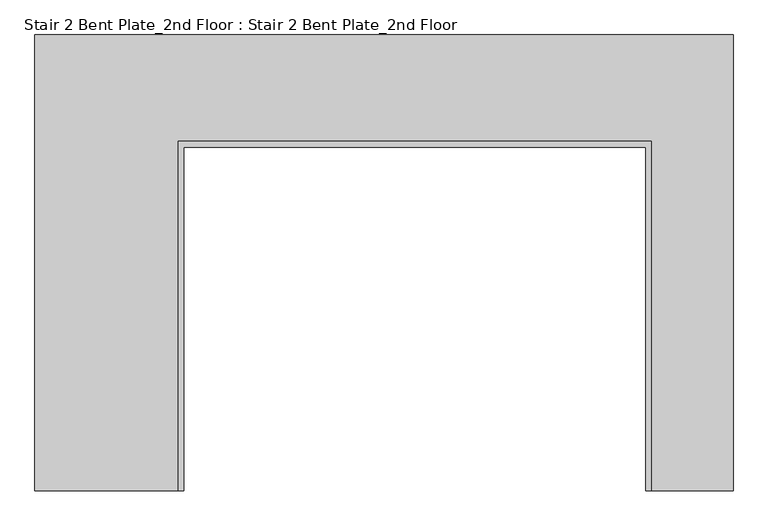
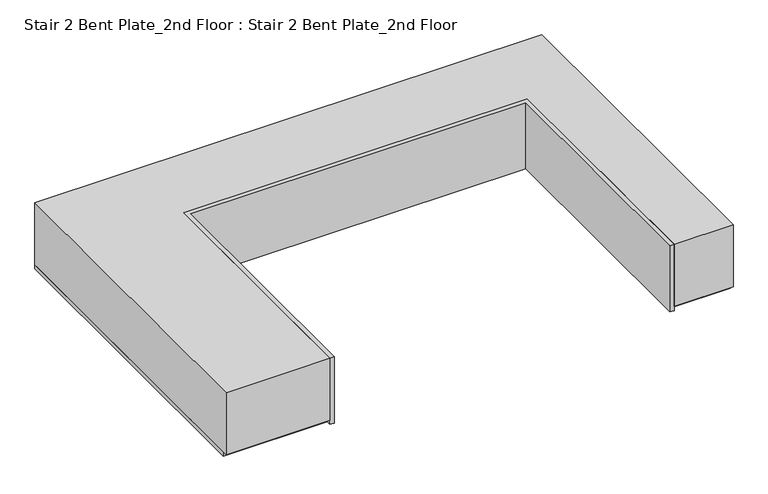
"""IFC4 building model written with IfcOpenShell, lengths in millimetres: proxy geometry, Stair 2 Bent Plate_2nd Floor : Stair 2 Bent Plate_2nd Floor."""

import ifcopenshell
import ifcopenshell.guid

model = None  # the IFC model being written
_history = None  # IfcOwnerHistory: only IFC2X3 demands one
_inside = {}  # id of a spatial element -> (the spatial element, [elements in it])
_under = {}  # id of a project, library or spatial element -> (it, [spatial elements below it])
_declared = {}  # id of a project -> (the project, [libraries it declares])
_typed = {}  # id of a type object -> (the type object, [elements of that type])
_made_of = {}  # id of a material, layer set ... -> (it, [elements and type objects made of it])


def new_model(schema):
    """Start an empty IFC model of exactly this schema.

    Asked for "IFC4X3", IfcOpenShell would pick the latest addendum, in which some entities
    have other attributes; the version numbers below select the first issue.
    IFC2X3 requires an IfcOwnerHistory on every rooted entity: one is made here for all.
    """
    global model, _history
    if schema == "IFC4X3":
        model = ifcopenshell.file(schema_version=(4, 3, 0, 0))
    else:
        model = ifcopenshell.file(schema=schema)
    _inside.clear()
    _under.clear()
    _declared.clear()
    _typed.clear()
    _made_of.clear()
    _history = None
    if model.schema == "IFC2X3":
        org = make("IfcOrganization", Name="unknown")
        user = make(
            "IfcPersonAndOrganization",
            ThePerson=make("IfcPerson", FamilyName="unknown"),
            TheOrganization=org,
        )
        app = make(
            "IfcApplication",
            ApplicationDeveloper=org,
            Version="unknown",
            ApplicationFullName="unknown",
            ApplicationIdentifier="unknown",
        )
        _history = make(
            "IfcOwnerHistory",
            OwningUser=user,
            OwningApplication=app,
            ChangeAction="ADDED",
            CreationDate=0,
        )
    return model


def make(cls, **values):
    """One entity of the class cls with the attributes given. An attribute that is None is left unset."""
    return model.create_entity(
        cls, **{name: value for name, value in values.items() if value is not None}
    )


def rooted(cls, **values):
    """An entity with a GlobalId (a new one), such as an element, a storey or a relation."""
    return make(cls, GlobalId=ifcopenshell.guid.new(), OwnerHistory=_history, **values)


def si_unit(unit_type, name, prefix=None):
    """IfcSIUnit, for example si_unit("LENGTHUNIT", "METRE", prefix="MILLI")."""
    return make("IfcSIUnit", UnitType=unit_type, Prefix=prefix, Name=name)


def assignment(units):
    """IfcUnitAssignment: the units of a project."""
    return None if units is None else make("IfcUnitAssignment", Units=units)


def point(xyz):
    """IfcCartesianPoint."""
    return None if xyz is None else make("IfcCartesianPoint", Coordinates=xyz)


def direction(xyz):
    """IfcDirection."""
    return None if xyz is None else make("IfcDirection", DirectionRatios=xyz)


def frame(location, z_axis=None, x_axis=None):
    """IfcAxis2Placement3D, a coordinate frame: its origin and axes. An axis left out is left unset."""
    return make(
        "IfcAxis2Placement3D",
        Location=point(location),
        Axis=direction(z_axis),
        RefDirection=direction(x_axis),
    )


def origin():
    """The frame at (0, 0, 0) with its axes left unset."""
    return frame((0.0, 0.0, 0.0))


def origin_with_axes():
    """The frame at (0, 0, 0) with the z axis (0, 0, 1) and the x axis (1, 0, 0) written out."""
    return frame((0.0, 0.0, 0.0), z_axis=(0.0, 0.0, 1.0), x_axis=(1.0, 0.0, 0.0))


def place(relative_to, where):
    """IfcLocalPlacement: puts the frame where relative to a parent placement (None: the world)."""
    return make(
        "IfcLocalPlacement", PlacementRelTo=relative_to, RelativePlacement=where
    )


def context(
    kind, dimensions, precision=None, world=None, true_north=None, identifier=None
):
    """IfcGeometricRepresentationContext, for example the 3D "Model" context."""
    return make(
        "IfcGeometricRepresentationContext",
        ContextIdentifier=identifier,
        ContextType=kind,
        CoordinateSpaceDimension=dimensions,
        Precision=precision,
        WorldCoordinateSystem=world,
        TrueNorth=true_north,
    )


def project(units=None, contexts=None):
    """IfcProject with its units and contexts."""
    return rooted(
        "IfcProject",
        Name="project",
        RepresentationContexts=contexts,
        UnitsInContext=assignment(units),
    )


def spatial(cls, under=None, at=None, **own):
    """A site, building, storey or space (cls), placed at a placement, below another one or the project."""
    s = rooted(cls, ObjectPlacement=at, **own)
    if under is not None:
        _under.setdefault(under.id(), (under, []))[1].append(s)
    return s


def polyline(points):
    """IfcPolyline through the points."""
    return make("IfcPolyline", Points=[point(p) for p in points])


def outline(outer, holes=None, kind="AREA"):
    """IfcArbitraryClosedProfileDef: a profile drawn as a closed curve; with holes, ...WithVoids."""
    if holes is None:
        return make("IfcArbitraryClosedProfileDef", ProfileType=kind, OuterCurve=outer)
    return make(
        "IfcArbitraryProfileDefWithVoids",
        ProfileType=kind,
        OuterCurve=outer,
        InnerCurves=holes,
    )


def extrude(swept, where, along, depth):
    """IfcExtrudedAreaSolid: the profile swept, set in the frame where, extruded along a direction by depth."""
    return make(
        "IfcExtrudedAreaSolid",
        SweptArea=swept,
        Position=where,
        ExtrudedDirection=direction(along),
        Depth=depth,
    )


def shape(context_of_items, identifier, shape_type, items):
    """IfcShapeRepresentation: the items that make up one representation, for example the "Body"."""
    return make(
        "IfcShapeRepresentation",
        ContextOfItems=context_of_items,
        RepresentationIdentifier=identifier,
        RepresentationType=shape_type,
        Items=items,
    )


def source(mapping_origin, context_of_items, identifier, shape_type, items):
    """IfcRepresentationMap: a shape defined once, which mapped items show again and again."""
    return make(
        "IfcRepresentationMap",
        MappingOrigin=mapping_origin,
        MappedRepresentation=shape(context_of_items, identifier, shape_type, items),
    )


def transform(
    local_origin,
    x_axis=None,
    y_axis=None,
    z_axis=None,
    scale=None,
    scale2=None,
    scale3=None,
    uniform=True,
):
    """IfcCartesianTransformationOperator3D, or its non-uniform kind. x_axis, y_axis, z_axis: its Axis1, 2, 3."""
    if uniform:
        return make(
            "IfcCartesianTransformationOperator3D",
            Axis1=direction(x_axis),
            Axis2=direction(y_axis),
            LocalOrigin=point(local_origin),
            Scale=scale,
            Axis3=direction(z_axis),
        )
    return make(
        "IfcCartesianTransformationOperator3DnonUniform",
        Axis1=direction(x_axis),
        Axis2=direction(y_axis),
        LocalOrigin=point(local_origin),
        Scale=scale,
        Axis3=direction(z_axis),
        Scale2=scale2,
        Scale3=scale3,
    )


def mapped(mapping_source, mapping_target):
    """IfcMappedItem: shows the shape of a source again, moved by a transform."""
    return make(
        "IfcMappedItem", MappingSource=mapping_source, MappingTarget=mapping_target
    )


def made_of(thing, what):
    """Note that an element or type object is made of a material, layer set ...; save() writes the relation."""
    if what is not None:
        _made_of.setdefault(what.id(), (what, []))[1].append(thing)
    return thing


def element(
    cls,
    number,
    at=None,
    inside=None,
    cuts=None,
    type_object=None,
    material=None,
    context=None,
    identifier="Body",
    shape_type=None,
    held_by="IfcProductDefinitionShape",
    body=None,
    shapes=None,
    **own,
):
    """One element of the class cls, such as IfcWall. Its Tag is "e" and its number.

    at: its placement. inside: the storey or other place that contains it. cuts: it is an
    opening in that element (IfcRelVoidsElement). A single representation is given by context,
    identifier, shape_type and body (its items); several are given by shapes. held_by: the class
    of the entity that holds the representations. save() writes the other relations.
    """
    e = rooted(cls, Tag="e%d" % number, ObjectPlacement=at, **own)
    if body is not None:
        shapes = [shape(context, identifier, shape_type, body)]
    if shapes is not None:
        e.Representation = make(held_by, Representations=shapes)
    if inside is not None:
        _inside.setdefault(inside.id(), (inside, []))[1].append(e)
    if cuts is not None:
        rooted(
            "IfcRelVoidsElement", RelatingBuildingElement=cuts, RelatedOpeningElement=e
        )
    if type_object is not None:
        _typed.setdefault(type_object.id(), (type_object, []))[1].append(e)
    return made_of(e, material)


def aggregate(whole, parts):
    """IfcRelAggregates: a whole, such as a stair, and the parts it consists of."""
    return rooted("IfcRelAggregates", RelatingObject=whole, RelatedObjects=parts)


def save(model, path):
    """Write the relations noted so far, then the file.

    IfcRelAggregates (storeys below a building ...), IfcRelContainedInSpatialStructure (elements
    in a storey), IfcRelDefinesByType, IfcRelAssociatesMaterial and IfcRelDeclares: one each for
    every whole, place, type object, material and project.
    """
    for whole, parts in _under.values():
        aggregate(whole, parts)
    for where, things in _inside.values():
        rooted(
            "IfcRelContainedInSpatialStructure",
            RelatedElements=things,
            RelatingStructure=where,
        )
    for kind, things in _typed.values():
        rooted("IfcRelDefinesByType", RelatedObjects=things, RelatingType=kind)
    for what, things in _made_of.values():
        rooted("IfcRelAssociatesMaterial", RelatedObjects=things, RelatingMaterial=what)
    for by, libraries in _declared.values():
        rooted("IfcRelDeclares", RelatingContext=by, RelatedDefinitions=libraries)
    model.write(path)


def stair_2_bent_plate_2nd_floor_stair_2_bent_plate_2nd_floor_d30ef73d(model_context):
    return source(origin(), model_context, "Body", "SweptSolid", [
        extrude(outline(polyline([(-314.325, -915.9875), (-314.325, 46.0375), (1158.875, 46.0375), (1158.875, -915.9875), (987.425, -915.9875), (987.425, -177.8), (-12.7, -177.8), (-12.7, -915.9875), (-314.325, -915.9875)])), frame((0.0, 0.0, 12.7), z_axis=(0.0, 0.0, 1.0), x_axis=(1.0, 0.0, 0.0)), (0.0, 0.0, 1.0), 190.5),
        extrude(outline(polyline([(-12.7, -901.7), (-314.325, -901.7), (-314.325, 46.0375), (1158.875, 46.0375), (1158.875, -901.7), (987.425, -901.7), (987.425, -177.8), (-12.7, -177.8), (-12.7, -901.7)])), origin_with_axes(), (0.0, 0.0, 1.0), 12.7),
        extrude(outline(polyline([(-12.7, -915.9875), (-12.7, -190.5), (-12.7, -177.8), (974.725, -177.8), (987.425, -177.8), (987.425, -915.9875), (974.725, -915.9875), (974.725, -190.5), (0.0, -190.5), (0.0, -915.9875), (-12.7, -915.9875)])), origin_with_axes(), (0.0, 0.0, 1.0), 203.2),
    ])


if __name__ == "__main__":
    model = new_model("IFC4")
    model_context = context("Model", 3, world=origin())
    ifc_project = project(units=[si_unit("LENGTHUNIT", "METRE", prefix="MILLI")], contexts=[model_context])
    site = spatial("IfcSite", under=ifc_project)
    building = spatial("IfcBuilding", under=site)
    placement = place(None, origin())
    stair_2_bent_plate_2nd_floor_stair_2_bent_plate_2nd_floor_shape = stair_2_bent_plate_2nd_floor_stair_2_bent_plate_2nd_floor_d30ef73d(model_context)
    element("IfcBuildingElementProxy", 1, Name="Stair 2 Bent Plate_2nd Floor : Stair 2 Bent Plate_2nd Floor", ObjectType="Stair 2 Bent Plate_2nd Floor : Stair 2 Bent Plate_2nd Floor", at=placement, inside=building, context=model_context, shape_type="MappedRepresentation", body=[
        mapped(stair_2_bent_plate_2nd_floor_stair_2_bent_plate_2nd_floor_shape, transform((0.0, 0.0, 0.0), x_axis=(1.0, 0.0, 0.0), y_axis=(0.0, 1.0, 0.0), z_axis=(0.0, 0.0, 1.0))),
    ])
    save(model, "model.ifc")

# Revit data of these elements
# Element 1 (IfcBuildingElementProxy, "Stair 2 Bent Plate_2nd Floor : Stair 2 Bent Plate_2nd Floor")
#   Materials on its faces: "Concrete Infill"
# Materials
#   "Concrete Infill": class "Generic", colour RGB 0 255 0, transparency 0, Cost = 0
